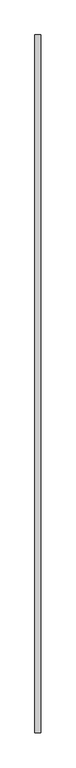
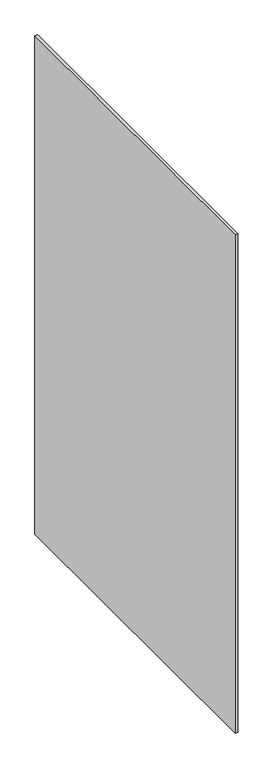
"""IFC4 building model written with IfcOpenShell, lengths in millimetres: proxy geometry, Generic Models 7:Generic Models 1:5:Generic Models 1:5 : Generic Models 7:Generic Models 1:337419:35 : Generic Models 7:Generic Models 1:5:Generic Models 1:5 : Generic Models 7:Generic Models 1:337419:311462."""

import ifcopenshell
import ifcopenshell.guid

model = None  # the IFC model being written
_history = None  # IfcOwnerHistory: only IFC2X3 demands one
_inside = {}  # id of a spatial element -> (the spatial element, [elements in it])
_under = {}  # id of a project, library or spatial element -> (it, [spatial elements below it])
_declared = {}  # id of a project -> (the project, [libraries it declares])
_typed = {}  # id of a type object -> (the type object, [elements of that type])
_made_of = {}  # id of a material, layer set ... -> (it, [elements and type objects made of it])


def new_model(schema):
    """Start an empty IFC model of exactly this schema.

    Asked for "IFC4X3", IfcOpenShell would pick the latest addendum, in which some entities
    have other attributes; the version numbers below select the first issue.
    IFC2X3 requires an IfcOwnerHistory on every rooted entity: one is made here for all.
    """
    global model, _history
    if schema == "IFC4X3":
        model = ifcopenshell.file(schema_version=(4, 3, 0, 0))
    else:
        model = ifcopenshell.file(schema=schema)
    _inside.clear()
    _under.clear()
    _declared.clear()
    _typed.clear()
    _made_of.clear()
    _history = None
    if model.schema == "IFC2X3":
        org = make("IfcOrganization", Name="unknown")
        user = make(
            "IfcPersonAndOrganization",
            ThePerson=make("IfcPerson", FamilyName="unknown"),
            TheOrganization=org,
        )
        app = make(
            "IfcApplication",
            ApplicationDeveloper=org,
            Version="unknown",
            ApplicationFullName="unknown",
            ApplicationIdentifier="unknown",
        )
        _history = make(
            "IfcOwnerHistory",
            OwningUser=user,
            OwningApplication=app,
            ChangeAction="ADDED",
            CreationDate=0,
        )
    return model


def make(cls, **values):
    """One entity of the class cls with the attributes given. An attribute that is None is left unset."""
    return model.create_entity(
        cls, **{name: value for name, value in values.items() if value is not None}
    )


def rooted(cls, **values):
    """An entity with a GlobalId (a new one), such as an element, a storey or a relation."""
    return make(cls, GlobalId=ifcopenshell.guid.new(), OwnerHistory=_history, **values)


def si_unit(unit_type, name, prefix=None):
    """IfcSIUnit, for example si_unit("LENGTHUNIT", "METRE", prefix="MILLI")."""
    return make("IfcSIUnit", UnitType=unit_type, Prefix=prefix, Name=name)


def assignment(units):
    """IfcUnitAssignment: the units of a project."""
    return None if units is None else make("IfcUnitAssignment", Units=units)


def point(xyz):
    """IfcCartesianPoint."""
    return None if xyz is None else make("IfcCartesianPoint", Coordinates=xyz)


def direction(xyz):
    """IfcDirection."""
    return None if xyz is None else make("IfcDirection", DirectionRatios=xyz)


def frame(location, z_axis=None, x_axis=None):
    """IfcAxis2Placement3D, a coordinate frame: its origin and axes. An axis left out is left unset."""
    return make(
        "IfcAxis2Placement3D",
        Location=point(location),
        Axis=direction(z_axis),
        RefDirection=direction(x_axis),
    )


def origin():
    """The frame at (0, 0, 0) with its axes left unset."""
    return frame((0.0, 0.0, 0.0))


def place(relative_to, where):
    """IfcLocalPlacement: puts the frame where relative to a parent placement (None: the world)."""
    return make(
        "IfcLocalPlacement", PlacementRelTo=relative_to, RelativePlacement=where
    )


def context(
    kind, dimensions, precision=None, world=None, true_north=None, identifier=None
):
    """IfcGeometricRepresentationContext, for example the 3D "Model" context."""
    return make(
        "IfcGeometricRepresentationContext",
        ContextIdentifier=identifier,
        ContextType=kind,
        CoordinateSpaceDimension=dimensions,
        Precision=precision,
        WorldCoordinateSystem=world,
        TrueNorth=true_north,
    )


def project(units=None, contexts=None):
    """IfcProject with its units and contexts."""
    return rooted(
        "IfcProject",
        Name="project",
        RepresentationContexts=contexts,
        UnitsInContext=assignment(units),
    )


def spatial(cls, under=None, at=None, **own):
    """A site, building, storey or space (cls), placed at a placement, below another one or the project."""
    s = rooted(cls, ObjectPlacement=at, **own)
    if under is not None:
        _under.setdefault(under.id(), (under, []))[1].append(s)
    return s


def polyline(points):
    """IfcPolyline through the points."""
    return make("IfcPolyline", Points=[point(p) for p in points])


def outline(outer, holes=None, kind="AREA"):
    """IfcArbitraryClosedProfileDef: a profile drawn as a closed curve; with holes, ...WithVoids."""
    if holes is None:
        return make("IfcArbitraryClosedProfileDef", ProfileType=kind, OuterCurve=outer)
    return make(
        "IfcArbitraryProfileDefWithVoids",
        ProfileType=kind,
        OuterCurve=outer,
        InnerCurves=holes,
    )


def extrude(swept, where, along, depth):
    """IfcExtrudedAreaSolid: the profile swept, set in the frame where, extruded along a direction by depth."""
    return make(
        "IfcExtrudedAreaSolid",
        SweptArea=swept,
        Position=where,
        ExtrudedDirection=direction(along),
        Depth=depth,
    )


def shape(context_of_items, identifier, shape_type, items):
    """IfcShapeRepresentation: the items that make up one representation, for example the "Body"."""
    return make(
        "IfcShapeRepresentation",
        ContextOfItems=context_of_items,
        RepresentationIdentifier=identifier,
        RepresentationType=shape_type,
        Items=items,
    )


def source(mapping_origin, context_of_items, identifier, shape_type, items):
    """IfcRepresentationMap: a shape defined once, which mapped items show again and again."""
    return make(
        "IfcRepresentationMap",
        MappingOrigin=mapping_origin,
        MappedRepresentation=shape(context_of_items, identifier, shape_type, items),
    )


def transform(
    local_origin,
    x_axis=None,
    y_axis=None,
    z_axis=None,
    scale=None,
    scale2=None,
    scale3=None,
    uniform=True,
):
    """IfcCartesianTransformationOperator3D, or its non-uniform kind. x_axis, y_axis, z_axis: its Axis1, 2, 3."""
    if uniform:
        return make(
            "IfcCartesianTransformationOperator3D",
            Axis1=direction(x_axis),
            Axis2=direction(y_axis),
            LocalOrigin=point(local_origin),
            Scale=scale,
            Axis3=direction(z_axis),
        )
    return make(
        "IfcCartesianTransformationOperator3DnonUniform",
        Axis1=direction(x_axis),
        Axis2=direction(y_axis),
        LocalOrigin=point(local_origin),
        Scale=scale,
        Axis3=direction(z_axis),
        Scale2=scale2,
        Scale3=scale3,
    )


def mapped(mapping_source, mapping_target):
    """IfcMappedItem: shows the shape of a source again, moved by a transform."""
    return make(
        "IfcMappedItem", MappingSource=mapping_source, MappingTarget=mapping_target
    )


def made_of(thing, what):
    """Note that an element or type object is made of a material, layer set ...; save() writes the relation."""
    if what is not None:
        _made_of.setdefault(what.id(), (what, []))[1].append(thing)
    return thing


def element(
    cls,
    number,
    at=None,
    inside=None,
    cuts=None,
    type_object=None,
    material=None,
    context=None,
    identifier="Body",
    shape_type=None,
    held_by="IfcProductDefinitionShape",
    body=None,
    shapes=None,
    **own,
):
    """One element of the class cls, such as IfcWall. Its Tag is "e" and its number.

    at: its placement. inside: the storey or other place that contains it. cuts: it is an
    opening in that element (IfcRelVoidsElement). A single representation is given by context,
    identifier, shape_type and body (its items); several are given by shapes. held_by: the class
    of the entity that holds the representations. save() writes the other relations.
    """
    e = rooted(cls, Tag="e%d" % number, ObjectPlacement=at, **own)
    if body is not None:
        shapes = [shape(context, identifier, shape_type, body)]
    if shapes is not None:
        e.Representation = make(held_by, Representations=shapes)
    if inside is not None:
        _inside.setdefault(inside.id(), (inside, []))[1].append(e)
    if cuts is not None:
        rooted(
            "IfcRelVoidsElement", RelatingBuildingElement=cuts, RelatedOpeningElement=e
        )
    if type_object is not None:
        _typed.setdefault(type_object.id(), (type_object, []))[1].append(e)
    return made_of(e, material)


def aggregate(whole, parts):
    """IfcRelAggregates: a whole, such as a stair, and the parts it consists of."""
    return rooted("IfcRelAggregates", RelatingObject=whole, RelatedObjects=parts)


def save(model, path):
    """Write the relations noted so far, then the file.

    IfcRelAggregates (storeys below a building ...), IfcRelContainedInSpatialStructure (elements
    in a storey), IfcRelDefinesByType, IfcRelAssociatesMaterial and IfcRelDeclares: one each for
    every whole, place, type object, material and project.
    """
    for whole, parts in _under.values():
        aggregate(whole, parts)
    for where, things in _inside.values():
        rooted(
            "IfcRelContainedInSpatialStructure",
            RelatedElements=things,
            RelatingStructure=where,
        )
    for kind, things in _typed.values():
        rooted("IfcRelDefinesByType", RelatedObjects=things, RelatingType=kind)
    for what, things in _made_of.values():
        rooted("IfcRelAssociatesMaterial", RelatedObjects=things, RelatingMaterial=what)
    for by, libraries in _declared.values():
        rooted("IfcRelDeclares", RelatingContext=by, RelatedDefinitions=libraries)
    model.write(path)


def generic_models_ae916259(model_context):
    return source(origin(), model_context, "Body", "SweptSolid", [
        extrude(outline(polyline([(30.4457208, 560327.5617239), (30.4457208, 560345.6378538), (88.8218888, 560345.6378538), (90.8175588, 560347.6335238), (3712.5974457, 560347.6335238), (3712.5974457, 560327.5617239), (30.4457208, 560327.5617239)])), frame((0.0, -545612.3913841, 0.0), z_axis=(0.0, 1.0, 0.0), x_axis=(0.0, 0.0, 1.0)), (0.0, 0.0, 1.0), 2423.0786989),
    ])


if __name__ == "__main__":
    model = new_model("IFC4")
    model_context = context("Model", 3, world=origin())
    ifc_project = project(units=[si_unit("LENGTHUNIT", "METRE", prefix="MILLI")], contexts=[model_context])
    site = spatial("IfcSite", under=ifc_project)
    building = spatial("IfcBuilding", under=site)
    placement = place(None, origin())
    generic_models_shape = generic_models_ae916259(model_context)
    element("IfcBuildingElementProxy", 1, Name="Generic Models 7:Generic Models 1:5:Generic Models 1:5 : Generic Models 7:Generic Models 1:337419:35 : Generic Models 7:Generic Models 1:5:Generic Models 1:5 : Generic Models 7:Generic Models 1:337419:311462", ObjectType="Generic Models 7:Generic Models 1:5:Generic Models 1:5 : Generic Models 7:Generic Models 1:337419:35 : Generic Models 7:Generic Models 1:5:Generic Models 1:5 : Generic Models 7:Generic Models 1:337419:311462", at=placement, inside=building, context=model_context, shape_type="MappedRepresentation", body=[
        mapped(generic_models_shape, transform((0.0, 0.0, 0.0), x_axis=(1.0, 0.0, 0.0), y_axis=(0.0, 1.0, 0.0), z_axis=(0.0, 0.0, 1.0))),
    ])
    save(model, "model.ifc")

# Revit data of these elements
# Type "Generic Models 7:Generic Models 1:5:Generic Models 1:5 : Generic Models 7:Generic Models 1:337419:35 : Generic Models 7:Generic Models 1:5:Generic Models 1:5 : Generic Models 7:Generic Models 1:337419:311462"
#   NameOverride = "Generic Models 7:Generic Models 1:5:Generic Models 1:5 : Generic Models 7:Generic Models 1:337419:311462"
#   ObjectTypeOverride = "Generic Models 1:5 : Generic Models 7:Generic Models 1:337419"
#   Reference = "Generic Models 1"
#   Tag = "311462"
# Element 1 (IfcBuildingElementProxy, "Generic Models 7:Generic Models 1:5:Generic Models 1:5 : Generic Models 7:Generic Models 1:337419:35 : Generic Models 7:Generic Models 1:5:Generic Models 1:5 : Generic Models 7:Generic Models 1:337419:311462")
#   Materials on its faces: "1\" MINERAL WOOL BOARD INSULATION - BLACK MAT FACER"
# Materials
#   "1\" MINERAL WOOL BOARD INSULATION - BLACK MAT FACER": class "Unassigned", colour RGB 205 188 106, transparency 0, Cost = 0
